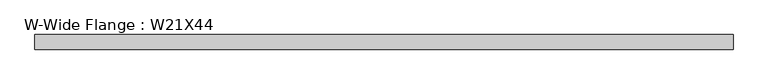
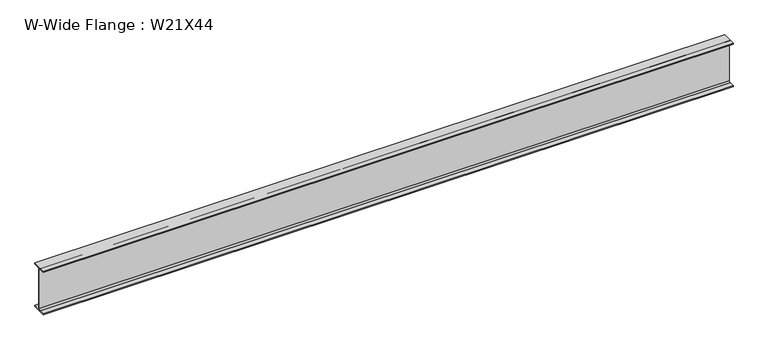
"""IFC4 building model written with IfcOpenShell, lengths in millimetres: beam geometry, W-Wide Flange : W21X44."""

from ifc_helpers import new_model, si_unit, point, frame, frame_2d, origin, place, context, project, spatial, polyline, circle_curve, trimmed, segment, composite_curve, outline, extrude, source, transform, mapped, element, save


def w_wide_flange_w21x44_bc81a974(model_context):
    return source(origin(), model_context, "Body", "SweptSolid", [
        extrude(outline(composite_curve([segment(polyline([(82.55, -251.46), (82.55, -262.89), (-82.55, -262.89), (-82.55, -251.46), (-21.59, -251.46)]), True, "CONTINUOUS"), segment(trimmed(circle_curve(frame_2d((-21.59, -234.315)), 17.145), [point((-21.59, -251.46))], [point((-4.445, -234.315))], True, "CARTESIAN"), True, "CONTINUOUS"), segment(polyline([(-4.445, -234.315), (-4.445, 234.315)]), True, "CONTINUOUS"), segment(trimmed(circle_curve(frame_2d((-21.59, 234.315)), 17.145), [point((-4.445, 234.315))], [point((-21.59, 251.46))], True, "CARTESIAN"), True, "CONTINUOUS"), segment(polyline([(-21.59, 251.46), (-82.55, 251.46), (-82.55, 262.89), (82.55, 262.89), (82.55, 251.46), (21.59, 251.46)]), True, "CONTINUOUS"), segment(trimmed(circle_curve(frame_2d((21.59, 234.315)), 17.145), [point((21.59, 251.46))], [point((4.445, 234.315))], True, "CARTESIAN"), True, "CONTINUOUS"), segment(polyline([(4.445, 234.315), (4.445, -234.315)]), True, "CONTINUOUS"), segment(trimmed(circle_curve(frame_2d((21.59, -234.315)), 17.145), [point((4.445, -234.315))], [point((21.59, -251.46))], True, "CARTESIAN"), True, "CONTINUOUS"), segment(polyline([(21.59, -251.46), (82.55, -251.46)]), True, "CONTINUOUS")], self_intersect=False)), frame((-3905.0724956, 0.0, 0.0), z_axis=(1.0, 0.0, 0.0), x_axis=(0.0, 1.0, 0.0)), (0.0, 0.0, 1.0), 7870.7248974),
    ])


if __name__ == "__main__":
    model = new_model("IFC4")
    model_context = context("Model", 3, world=origin())
    ifc_project = project(units=[si_unit("LENGTHUNIT", "METRE", prefix="MILLI")], contexts=[model_context])
    site = spatial("IfcSite", under=ifc_project)
    building = spatial("IfcBuilding", under=site)
    placement = place(None, origin())
    w_wide_flange_w21x44_shape = w_wide_flange_w21x44_bc81a974(model_context)
    element("IfcBeam", 1, ObjectType="W-Wide Flange : W21X44", at=placement, inside=building, context=model_context, shape_type="MappedRepresentation", body=[
        mapped(w_wide_flange_w21x44_shape, transform((0.0, 0.0, 0.0), x_axis=(1.0, 0.0, 0.0), y_axis=(0.0, 1.0, 0.0), z_axis=(0.0, 0.0, 1.0))),
    ])
    save(model, "model.ifc")

# Revit data of these elements
# Type "W-Wide Flange : W21X44"
#   Assembly Code = "B10"
#   W = 44
#   Length [instance default] = 1524 mm
#   bf = 165.1 mm
#   d = 525.78 mm
#   k = 28.575 mm
#   k2 = 17.145 mm
#   tf = 11.43 mm
#   tw = 8.89 mm
#   A = 0.00838708 m²
#   Structural Material [instance default] = Steel ASTM A992
# Element 1 (IfcBeam, "W-Wide Flange : W21X44")
#   Structural Material = Aluminum, Anodized Red
#   Materials on its faces: "Aluminum, Anodized Red"
# Materials
#   "Steel ASTM A992": class "Metal", colour RGB 128 0 0, transparency 0, Description = "Structural steel 50ksi", Cost = 0
#   "Aluminum, Anodized Red": class "Metal", colour RGB 120 120 120, transparency 0, Description = "Anodized aluminum, red", Cost = 0
